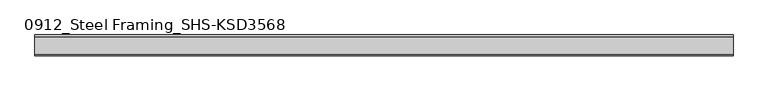
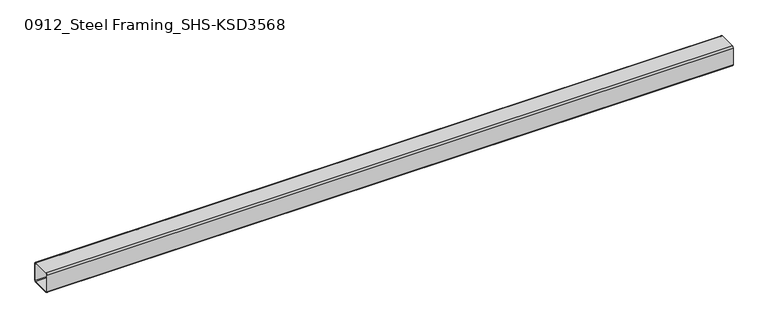
"""IFC4 building model written with IfcOpenShell, lengths in millimetres: beam geometry, 0912_Steel Framing_SHS-KSD3568 : H_SB_ASB_SHS-150x150x6."""

from ifc_helpers import new_model, si_unit, point, frame, frame_2d, origin, place, context, project, spatial, polyline, circle_curve, trimmed, segment, composite_curve, outline, extrude, source, transform, mapped, element, save


def beam_0912_steel_framing_shs_ksd3568_d3de1d54(model_context):
    return source(origin(), model_context, "Body", "SweptSolid", [
        extrude(outline(composite_curve([segment(polyline([(75.0, 63.0), (75.0, -63.0)]), True, "CONTINUOUS"), segment(trimmed(circle_curve(frame_2d((63.0, -63.0)), 12.0), [point((75.0, -63.0))], [point((63.0, -75.0))], False, "CARTESIAN"), True, "CONTINUOUS"), segment(polyline([(63.0, -75.0), (-63.0, -75.0)]), True, "CONTINUOUS"), segment(trimmed(circle_curve(frame_2d((-63.0, -63.0)), 12.0), [point((-63.0, -75.0))], [point((-75.0, -63.0))], False, "CARTESIAN"), True, "CONTINUOUS"), segment(polyline([(-75.0, -63.0), (-75.0, 63.0)]), True, "CONTINUOUS"), segment(trimmed(circle_curve(frame_2d((-63.0, 63.0)), 12.0), [point((-75.0, 63.0))], [point((-63.0, 75.0))], False, "CARTESIAN"), True, "CONTINUOUS"), segment(polyline([(-63.0, 75.0), (63.0, 75.0)]), True, "CONTINUOUS"), segment(trimmed(circle_curve(frame_2d((63.0, 63.0)), 12.0), [point((63.0, 75.0))], [point((75.0, 63.0))], False, "CARTESIAN"), True, "CONTINUOUS")], self_intersect=False), holes=[composite_curve([segment(trimmed(circle_curve(frame_2d((-63.0, 63.0)), 6.0), [point((-63.0, 69.0))], [point((-69.0, 63.0))], True, "CARTESIAN"), True, "CONTINUOUS"), segment(polyline([(-69.0, 63.0), (-69.0, -63.0)]), True, "CONTINUOUS"), segment(trimmed(circle_curve(frame_2d((-63.0, -63.0)), 6.0), [point((-69.0, -63.0))], [point((-63.0, -69.0))], True, "CARTESIAN"), True, "CONTINUOUS"), segment(polyline([(-63.0, -69.0), (63.0, -69.0)]), True, "CONTINUOUS"), segment(trimmed(circle_curve(frame_2d((63.0, -63.0)), 6.0), [point((63.0, -69.0))], [point((69.0, -63.0))], True, "CARTESIAN"), True, "CONTINUOUS"), segment(polyline([(69.0, -63.0), (69.0, 63.0)]), True, "CONTINUOUS"), segment(trimmed(circle_curve(frame_2d((63.0, 63.0)), 6.0), [point((69.0, 63.0))], [point((63.0, 69.0))], True, "CARTESIAN"), True, "CONTINUOUS"), segment(polyline([(63.0, 69.0), (-63.0, 69.0)]), True, "CONTINUOUS")], self_intersect=False)]), frame((-2490.0, 0.0, 0.0), z_axis=(1.0, 0.0, 0.0), x_axis=(0.0, 1.0, 0.0)), (0.0, 0.0, 1.0), 4980.0),
    ])


if __name__ == "__main__":
    model = new_model("IFC4")
    model_context = context("Model", 3, world=origin())
    ifc_project = project(units=[si_unit("LENGTHUNIT", "METRE", prefix="MILLI")], contexts=[model_context])
    site = spatial("IfcSite", under=ifc_project)
    building = spatial("IfcBuilding", under=site)
    placement = place(None, origin())
    beam_0912_steel_framing_shs_ksd3568_shape = beam_0912_steel_framing_shs_ksd3568_d3de1d54(model_context)
    element("IfcBeam", 1, ObjectType="0912_Steel Framing_SHS-KSD3568 : H_SB_ASB_SHS-150x150x6", at=placement, inside=building, context=model_context, shape_type="MappedRepresentation", body=[
        mapped(beam_0912_steel_framing_shs_ksd3568_shape, transform((0.0, 0.0, 0.0), x_axis=(1.0, 0.0, 0.0), y_axis=(0.0, 1.0, 0.0), z_axis=(0.0, 0.0, 1.0))),
    ])
    save(model, "model.ifc")

# Revit data of these elements
# Type "0912_Steel Framing_SHS-KSD3568 : H_SB_ASB_SHS-150x150x6"
#   H_WM Code_1 = "S01AA002-00001 | Main Steel Structure Fabrication Work | Shelter/Building | Medium Steel - Standard (90KG/M>Weight≥30KG/M) | Material: (   )"
#   H_WM Code_2 = "S03AA028-00001 | Main Steel Structure Erection Work | Shelter/Building | Medium Steel (90KG/M>Weight≥30KG/M) | Material: (   )"
#   H_WM Code_3 = "S01AA010-00001 | Main Steel Structure Fabrication Work | Shelter/Building | Steel Painting/Coating | for Non-Fireproofed Steel Surface, Surface Preparation, Primer, Second & Final Coat | Material: (   )"
#   H_Q'ty Cal Type Tag = "SB-Q2"
#   Perimeter = 0.60 m²/m
#   Nominal Weight = 26.40 kgf/m
#   Length [instance default] = 1.0000 m
#   b = 0.1500 m
#   h = 0.1500 m
#   tr = 0.0120 m
#   t = 0.0060 m
#   A = 28.36 m²
#   Structural Material [instance default] = Steel, 45-345
# Element 1 (IfcBeam, "0912_Steel Framing_SHS-KSD3568 : H_SB_ASB_SHS-150x150x6")
#   Structural Material = none
# Materials
#   "Steel, 45-345": class "Metal", colour RGB 189 187 185, transparency 0, Description = "Steel 345 MPa", Cost = 0
